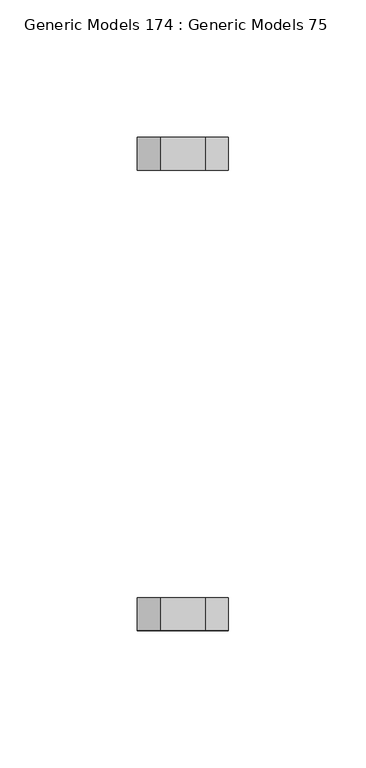
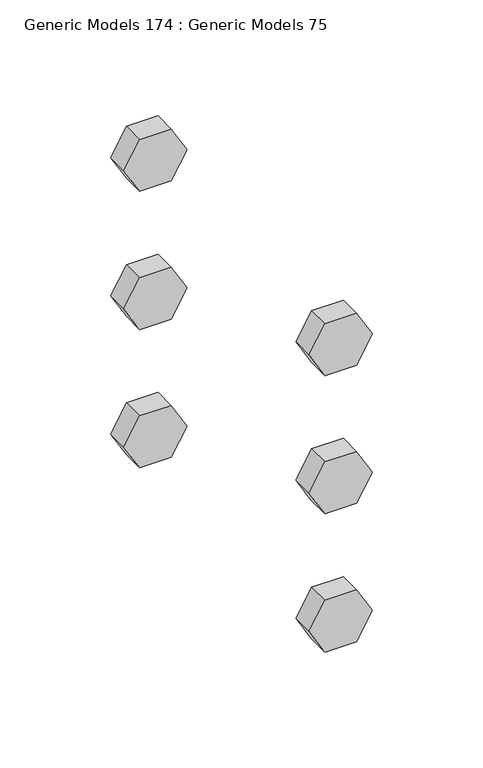
"""IFC4 building model written with IfcOpenShell, lengths in millimetres: proxy geometry, Generic Models 174 : Generic Models 75."""

from ifc_helpers import new_model, si_unit, frame, origin, place, context, project, spatial, polyline, outline, extrude, source, transform, mapped, element, save


def generic_models_174_generic_models_75_63e9463d(model_context):
    return source(origin(), model_context, "Body", "SweptSolid", [
        extrude(outline(polyline([(272027.8220065, 31970.0362939), (272013.5345065, 31978.2851858), (272013.5345065, 31994.7829698), (272027.8220065, 32003.0318618), (272042.1095065, 31994.7829698), (272042.1095065, 31978.2851858), (272027.8220065, 31970.0362939)])), frame((0.0, 30684.6469112, 0.0), z_axis=(0.0, 1.0, 0.0), x_axis=(0.0, 0.0, 1.0)), (0.0, 0.0, 1.0), 11.90625),
        extrude(outline(polyline([(272027.8220065, 31970.0362939), (272013.5345065, 31978.2851858), (272013.5345065, 31994.7829698), (272027.8220065, 32003.0318618), (272042.1095065, 31994.7829698), (272042.1095065, 31978.2851858), (272027.8220065, 31970.0362939)])), frame((0.0, 30852.1281612, 0.0), z_axis=(0.0, 1.0, 0.0), x_axis=(0.0, 0.0, 1.0)), (0.0, 0.0, 1.0), 11.90625),
        extrude(outline(polyline([(271951.6220065, 31970.0362939), (271937.3345065, 31978.2851858), (271937.3345065, 31994.7829698), (271951.6220065, 32003.0318618), (271965.9095065, 31994.7829698), (271965.9095065, 31978.2851858), (271951.6220065, 31970.0362939)])), frame((0.0, 30684.6469112, 0.0), z_axis=(0.0, 1.0, 0.0), x_axis=(0.0, 0.0, 1.0)), (0.0, 0.0, 1.0), 11.90625),
        extrude(outline(polyline([(271951.6220065, 31970.0362939), (271937.3345065, 31978.2851858), (271937.3345065, 31994.7829698), (271951.6220065, 32003.0318618), (271965.9095065, 31994.7829698), (271965.9095065, 31978.2851858), (271951.6220065, 31970.0362939)])), frame((0.0, 30852.1281612, 0.0), z_axis=(0.0, 1.0, 0.0), x_axis=(0.0, 0.0, 1.0)), (0.0, 0.0, 1.0), 11.90625),
        extrude(outline(polyline([(271875.4220065, 31970.0362939), (271861.1345065, 31978.2851858), (271861.1345065, 31994.7829698), (271875.4220065, 32003.0318618), (271889.7095065, 31994.7829698), (271889.7095065, 31978.2851858), (271875.4220065, 31970.0362939)])), frame((0.0, 30684.6469112, 0.0), z_axis=(0.0, 1.0, 0.0), x_axis=(0.0, 0.0, 1.0)), (0.0, 0.0, 1.0), 11.90625),
        extrude(outline(polyline([(271875.4220065, 31970.0362939), (271861.1345065, 31978.2851858), (271861.1345065, 31994.7829698), (271875.4220065, 32003.0318618), (271889.7095065, 31994.7829698), (271889.7095065, 31978.2851858), (271875.4220065, 31970.0362939)])), frame((0.0, 30852.1281612, 0.0), z_axis=(0.0, 1.0, 0.0), x_axis=(0.0, 0.0, 1.0)), (0.0, 0.0, 1.0), 11.90625),
    ])


if __name__ == "__main__":
    model = new_model("IFC4")
    model_context = context("Model", 3, world=origin())
    ifc_project = project(units=[si_unit("LENGTHUNIT", "METRE", prefix="MILLI")], contexts=[model_context])
    site = spatial("IfcSite", under=ifc_project)
    building = spatial("IfcBuilding", under=site)
    placement = place(None, origin())
    generic_models_174_generic_models_75_shape = generic_models_174_generic_models_75_63e9463d(model_context)
    element("IfcBuildingElementProxy", 1, Name="Generic Models 174 : Generic Models 75", ObjectType="Generic Models 174 : Generic Models 75", at=placement, inside=building, context=model_context, shape_type="MappedRepresentation", body=[
        mapped(generic_models_174_generic_models_75_shape, transform((0.0, 0.0, 0.0), x_axis=(1.0, 0.0, 0.0), y_axis=(0.0, 1.0, 0.0), z_axis=(0.0, 0.0, 1.0))),
    ])
    save(model, "model.ifc")

# Revit data of these elements
# Element 1 (IfcBuildingElementProxy, "Generic Models 174 : Generic Models 75")
#   Materials on its faces: "3/4\" GALV. THRU BOLTS"
# Materials
#   "3/4\" GALV. THRU BOLTS": class "Generic", colour RGB 105 69 171, transparency 0, Cost = 0
